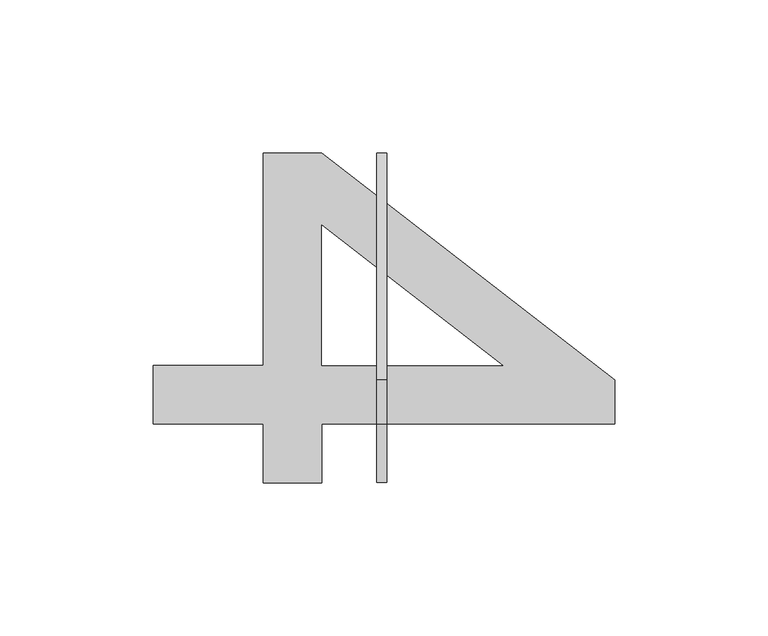
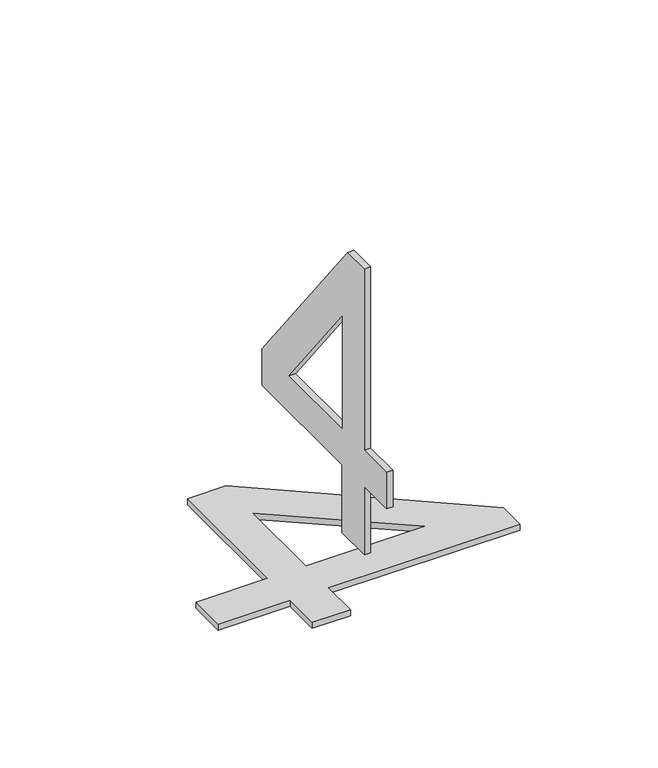
"""IFC4 building model written with IfcOpenShell, lengths in millimetres: proxy geometry, Grid Number2_FedEx : Grid Number2_FedEx."""

from ifc_helpers import new_model, si_unit, frame, origin, origin_with_axes, place, context, project, spatial, polyline, outline, extrude, source, transform, mapped, element, save


def entourage_280100bd(model_context):
    return source(origin(), model_context, "Body", "SweptSolid", [
        extrude(outline(polyline([(-184.2739267, 209.3640392), (-148.3921885, 209.3640392), (-148.3921885, 278.7353998), (-129.2552614, 278.7353998), (-33.570626, 204.5798074), (-33.570626, 190.2271121), (-129.2552614, 190.2271121), (-129.2552614, 171.090185), (-148.3921885, 171.090185), (-148.3921885, 190.2271121), (-184.2739267, 190.2271121), (-184.2739267, 209.3640392)]), holes=[polyline([(-129.2552614, 209.3640392), (-70.1251468, 209.3640392), (-129.2552614, 255.1880091), (-129.2552614, 209.3640392)])]), origin_with_axes(), (0.0, 0.0, 1.0), 3.175),
        extrude(outline(polyline([(209.3640392, 14.2382753), (190.2271121, 14.2382753), (190.2271121, 50.1200136), (171.090185, 50.1200136), (171.090185, 69.2569407), (190.2271121, 69.2569407), (190.2271121, 164.9415761), (204.5798074, 164.9415761), (278.7353998, 69.2569407), (278.7353998, 50.1200136), (209.3640392, 50.1200136), (209.3640392, 14.2382753)]), holes=[polyline([(209.3640392, 69.2569407), (255.1880091, 69.2569407), (209.3640392, 128.3870552), (209.3640392, 69.2569407)])]), frame((-111.2489267, 0.0, 0.0), z_axis=(1.0, 0.0, 0.0), x_axis=(0.0, 1.0, 0.0)), (0.0, 0.0, 1.0), 3.175),
    ])


if __name__ == "__main__":
    model = new_model("IFC4")
    model_context = context("Model", 3, world=origin())
    ifc_project = project(units=[si_unit("LENGTHUNIT", "METRE", prefix="MILLI")], contexts=[model_context])
    site = spatial("IfcSite", under=ifc_project)
    building = spatial("IfcBuilding", under=site)
    placement = place(None, origin())
    entourage_shape = entourage_280100bd(model_context)
    element("IfcBuildingElementProxy", 1, Name="Grid Number2_FedEx : Grid Number2_FedEx", ObjectType="Grid Number2_FedEx : Grid Number2_FedEx", at=placement, inside=building, context=model_context, shape_type="MappedRepresentation", body=[
        mapped(entourage_shape, transform((0.0, 0.0, 0.0), x_axis=(1.0, 0.0, 0.0), y_axis=(0.0, 1.0, 0.0), z_axis=(0.0, 0.0, 1.0))),
    ])
    save(model, "model.ifc")

# Revit data of these elements
# Type "Grid Number2_FedEx : Grid Number2_FedEx"
#   Grid [instance default] = "S"
#   Label Width [instance default] = 1' - 0"
#   Half Box Width2 [instance default] = 0' - 6.13846"
#   Half Box Width [instance default] = 0' - 6"
#   Robust [instance default] = yes
#   Height = 0
#   Assembly Code = ""
# Element 1 (IfcBuildingElementProxy, "Grid Number2_FedEx : Grid Number2_FedEx")
#   Grid = "4"
#   Robust = no
#   Materials on its faces: "Letter"
# Materials
#   "Letter": class "Unassigned", colour RGB 178 187 30, transparency 0, Comments = "Rendering appearance not upgraded "
